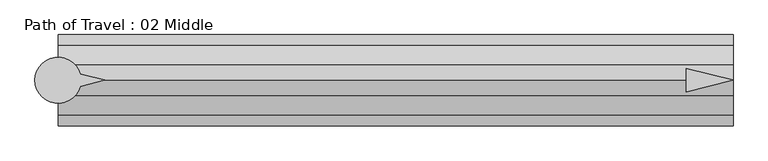
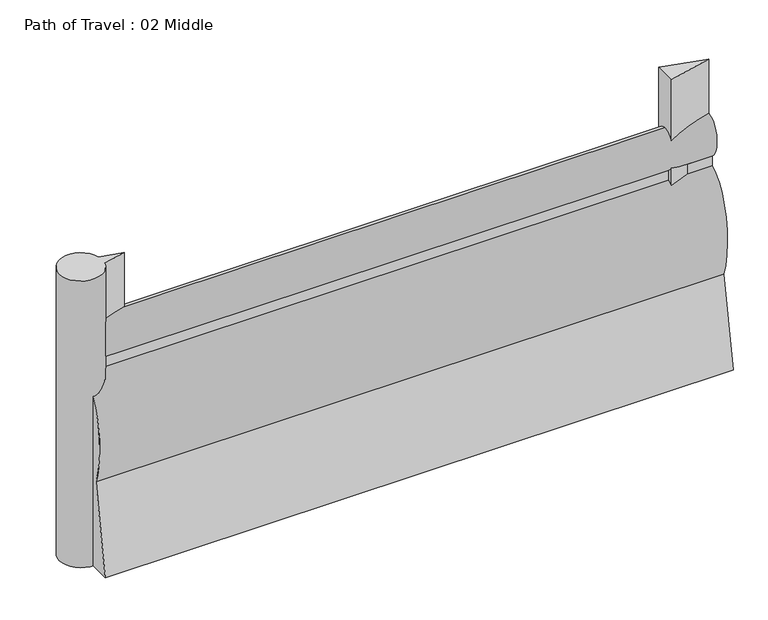
"""IFC4 building model written with IfcOpenShell, lengths in millimetres: proxy geometry, Path of Travel : 02 Middle."""

from ifc_helpers import new_model, si_unit, point, frame, frame_2d, origin, origin_with_axes, place, context, project, spatial, polyline, circle_curve, ellipse_curve, trimmed, segment, composite_curve, outline, extrude, source, transform, mapped, element, save
from ifc_brep_helpers import plane_surface, extruded_surface, advanced_brep


def path_of_travel_02_middle_5bade7f2(model_context):
    return source(origin(), model_context, "Body", "SolidModel", [
        advanced_brep(
        [(227.5554837, 0.0, 1727.2), (227.5554837, 42.9018657, 1436.6534209), (227.5554837, 42.9018657, 1363.4763406), (227.5554837, 184.1186263, 643.4144547), (227.5554837, 297.5699544, 0.0), (227.5554837, 145.6574193, 0.0), (227.5554837, 0.0, 584.2), (227.5554837, -145.6574193, 0.0), (227.5554837, -297.5699544, 0.0), (227.5554837, -184.1186263, 643.4144547), (227.5554837, -42.9018657, 1363.4763406), (227.5554837, -42.9018657, 1436.6534209), (4635.9128813, 0.0, 1727.2), (4635.9128813, -42.9018657, 1436.6534209), (4635.9128813, -42.9018657, 1363.4763406), (4635.9128813, -184.1186263, 643.4144547), (4635.9128813, -297.5699544, 0.0), (4635.9128813, -145.6574193, 0.0), (4635.9128813, 0.0, 584.2), (4635.9128813, 145.6574193, 0.0), (4635.9128813, 297.5699544, 0.0), (4635.9128813, 184.1186263, 643.4144547), (4635.9128813, 42.9018657, 1363.4763406), (4635.9128813, 42.9018657, 1436.6534209)],
        [
            (0, 1, ellipse_curve(frame((227.5554837, 0.0, 1574.8), z_axis=(-1.0, 0.0, 0.0), x_axis=(0.0, 0.0, 1.0)), 152.4, 101.6)),
            (1, 2),
            (2, 3, ellipse_curve(frame((227.5554837, 0.0, 914.4), z_axis=(-1.0, 0.0, 0.0), x_axis=(0.0, 0.0, -1.0)), 457.2, 228.6)),
            (3, 4),
            (4, 5),
            (5, 6),
            (6, 7),
            (7, 8),
            (8, 9),
            (9, 10, ellipse_curve(frame((227.5554837, 0.0, 914.4), z_axis=(-1.0, 0.0, 0.0), x_axis=(0.0, 0.0, -1.0)), 457.2, 228.6)),
            (10, 11),
            (11, 0, ellipse_curve(frame((227.5554837, 0.0, 1574.8), z_axis=(-1.0, 0.0, 0.0), x_axis=(0.0, 0.0, 1.0)), 152.4, 101.6)),
            (12, 13, ellipse_curve(frame((4635.9128813, 0.0, 1574.8), z_axis=(1.0, 0.0, 0.0), x_axis=(0.0, 0.0, 1.0)), 152.4, 101.6)),
            (13, 14),
            (14, 15, ellipse_curve(frame((4635.9128813, 0.0, 914.4), z_axis=(1.0, 0.0, 0.0), x_axis=(0.0, 0.0, -1.0)), 457.2, 228.6)),
            (15, 16),
            (16, 17),
            (17, 18),
            (18, 19),
            (19, 20),
            (20, 21),
            (21, 22, ellipse_curve(frame((4635.9128813, 0.0, 914.4), z_axis=(1.0, 0.0, 0.0), x_axis=(0.0, 0.0, -1.0)), 457.2, 228.6)),
            (22, 23),
            (23, 12, ellipse_curve(frame((4635.9128813, 0.0, 1574.8), z_axis=(1.0, 0.0, 0.0), x_axis=(0.0, 0.0, 1.0)), 152.4, 101.6)),
            (0, 12),
            (23, 1),
            (22, 2),
            (21, 3),
            (20, 4),
            (19, 5),
            (18, 6),
            (17, 7),
            (16, 8),
            (15, 9),
            (14, 10),
            (13, 11),
        ],
        [
            plane_surface(frame((227.5554837, 0.0, 0.0), z_axis=(-1.0, 0.0, 0.0), x_axis=(0.0, 0.0, 1.0))),
            plane_surface(frame((4635.9128813, 0.0, 0.0), z_axis=(1.0, 0.0, 0.0), x_axis=(0.0, 0.0, 1.0))),
            extruded_surface(trimmed(ellipse_curve(frame((4635.9128813, 0.0, 1574.8), z_axis=(-1.0, 0.0, 0.0), x_axis=(0.0, 0.0, 1.0)), 152.4, 101.6), [point((4635.9128813, 0.0, 1727.2))], [point((4635.9128813, 42.9018657, 1436.6534209))], True, "CARTESIAN"), (-4408.3573976, 0.0, 0.0), 4408.3573976),
            plane_surface(frame((227.5554837, 42.9018657, 1436.6534209), z_axis=(0.0, 1.0, 0.0), x_axis=(1.0, 0.0, 0.0))),
            extruded_surface(trimmed(ellipse_curve(frame((4635.9128813, 0.0, 914.4), z_axis=(-1.0, 0.0, 0.0), x_axis=(0.0, 0.0, -1.0)), 457.2, 228.6), [point((4635.9128813, 42.9018657, 1363.4763406))], [point((4635.9128813, 184.1186263, 643.4144547))], True, "CARTESIAN"), (-4408.3573976, 0.0, 0.0), 4408.3573976),
            plane_surface(frame((227.5554837, 184.1186263, 643.4144547), z_axis=(0.0, 0.9848077530122078, 0.1736481776669322), x_axis=(1.0, 0.0, 0.0))),
            plane_surface(frame((227.5554837, 297.5699544, 0.0), z_axis=(0.0, 0.0, -1.0), x_axis=(1.0, 0.0, 0.0))),
            plane_surface(frame((227.5554837, 145.6574193, 0.0), z_axis=(0.0, -0.9702957262760199, -0.2419218955995739), x_axis=(1.0, 0.0, 0.0))),
            plane_surface(frame((227.5554837, 0.0, 584.2), z_axis=(0.0, 0.9702957262759961, -0.24192189559966923), x_axis=(1.0, 0.0, 0.0))),
            plane_surface(frame((227.5554837, -145.6574193, 0.0), z_axis=(0.0, 0.0, -1.0), x_axis=(1.0, 0.0, 0.0))),
            plane_surface(frame((227.5554837, -297.5699544, 0.0), z_axis=(0.0, -0.984807753012208, 0.17364817766693066), x_axis=(1.0, 0.0, 0.0))),
            extruded_surface(trimmed(ellipse_curve(frame((4635.9128813, 0.0, 914.4), z_axis=(-1.0, 0.0, 0.0), x_axis=(0.0, 0.0, -1.0)), 457.2, 228.6), [point((4635.9128813, -184.1186263, 643.4144547))], [point((4635.9128813, -42.9018657, 1363.4763406))], True, "CARTESIAN"), (-4408.3573976, 0.0, 0.0), 4408.3573976),
            plane_surface(frame((227.5554837, -42.9018657, 1363.4763406), z_axis=(0.0, -1.0, 0.0), x_axis=(1.0, 0.0, 0.0))),
            extruded_surface(trimmed(ellipse_curve(frame((4635.9128813, 0.0, 1574.8), z_axis=(-1.0, 0.0, 0.0), x_axis=(0.0, 0.0, 1.0)), 152.4, 101.6), [point((4635.9128813, -42.9018657, 1436.6534209))], [point((4635.9128813, 0.0, 1727.2))], True, "CARTESIAN"), (-4408.3573976, 0.0, 0.0), 4408.3573976),
        ],
        [
            (0, [[1, 2, 3, 4, 5, 6, 7, 8, 9, 10, 11, 12]]),
            (1, [[13, 14, 15, 16, 17, 18, 19, 20, 21, 22, 23, 24]]),
            (2, [[-1, 25, -24, 26]]),
            (3, [[-2, -26, -23, 27]]),
            (4, [[-3, -27, -22, 28]]),
            (5, [[-4, -28, -21, 29]]),
            (6, [[-5, -29, -20, 30]]),
            (7, [[-6, -30, -19, 31]]),
            (8, [[-7, -31, -18, 32]]),
            (9, [[-8, -32, -17, 33]]),
            (10, [[-9, -33, -16, 34]]),
            (11, [[-10, -34, -15, 35]]),
            (12, [[-11, -35, -14, 36]]),
            (13, [[-12, -36, -13, -25]]),
        ],
    ),
        extrude(outline(polyline([(4329.9077347, 76.2006338), (4635.9128813, 0.0), (4329.9077347, -76.2006338), (4329.9077347, 76.2006338)])), origin_with_axes(), (0.0, 0.0, 1.0), 2129.5973753),
        extrude(outline(composite_curve([segment(polyline([(372.7837828, 39.4440225), (531.182385, 0.0), (372.7837828, -39.4440225)]), True, "CONTINUOUS"), segment(trimmed(circle_curve(frame_2d((227.2200886, 0.0)), 150.8131956), [point((372.7837828, -39.4440225))], [point((372.7837828, 39.4440225))], False, "CARTESIAN"), True, "CONTINUOUS")], self_intersect=False)), origin_with_axes(), (0.0, 0.0, 1.0), 2129.5973753),
    ])


if __name__ == "__main__":
    model = new_model("IFC4")
    model_context = context("Model", 3, world=origin())
    ifc_project = project(units=[si_unit("LENGTHUNIT", "METRE", prefix="MILLI")], contexts=[model_context])
    site = spatial("IfcSite", under=ifc_project)
    building = spatial("IfcBuilding", under=site)
    placement = place(None, origin())
    path_of_travel_02_middle_shape = path_of_travel_02_middle_5bade7f2(model_context)
    element("IfcBuildingElementProxy", 1, Name="Path of Travel : 02 Middle", ObjectType="Path of Travel : 02 Middle", at=placement, inside=building, context=model_context, shape_type="MappedRepresentation", body=[
        mapped(path_of_travel_02_middle_shape, transform((0.0, 0.0, 0.0), x_axis=(1.0, 0.0, 0.0), y_axis=(0.0, 1.0, 0.0), z_axis=(0.0, 0.0, 1.0))),
    ])
    save(model, "model.ifc")

# Revit data of these elements
# Type "Path of Travel : 02 Middle"
#   Path of Egress [instance default] = 4' - 0"
#   built-in parameter 1001306 [instance default] = 4 (stored number, unit not read)
#   Dot at Start = no
#   Arrow in Middle = yes
#   Arrow at End = no
#   Egress Path = none
# Element 1 (IfcBuildingElementProxy, "Path of Travel : 02 Middle")
#   Path of Egress = 14' - 5.55738"
#   built-in parameter 1001306 = 14.4631 (stored number, unit not read)
#   Materials on its faces: "Egress Path Solid", "solid"
# Materials
#   "Egress Path Solid": class "Unassigned", colour RGB 255 128 64, transparency 0.75, Comments = "Rendering appearance not upgraded "
#   "solid": class "Generic", colour RGB 120 120 120, transparency 0, Cost = 0
